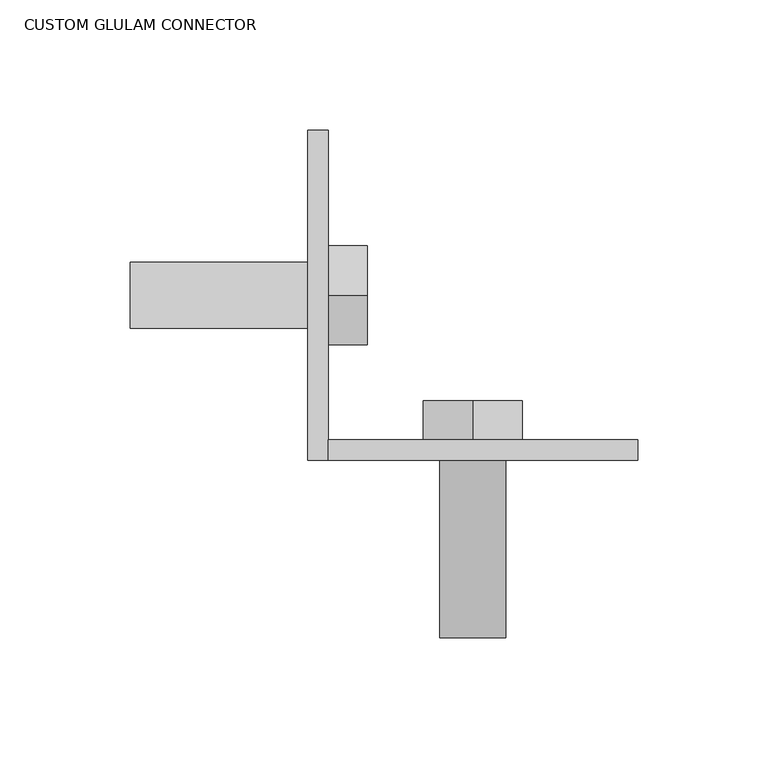
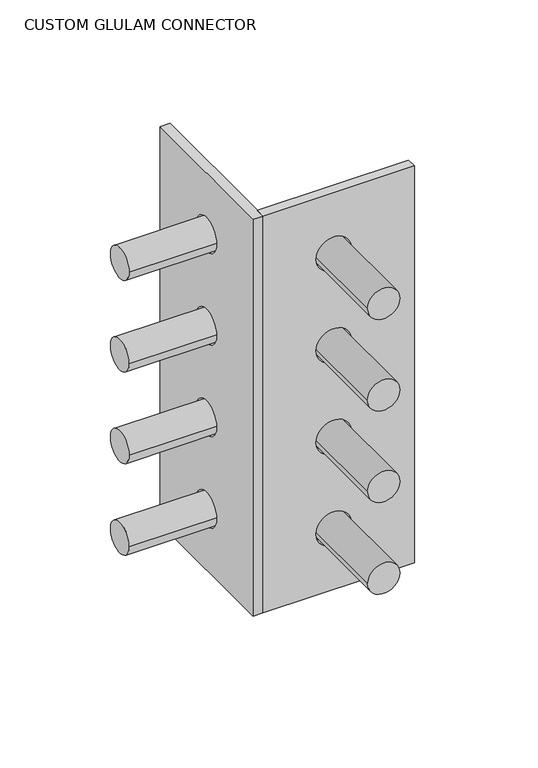
"""IFC4 building model written with IfcOpenShell, lengths in millimetres: fastener geometry, CUSTOM GLULAM CONNECTOR."""

from ifc_helpers import new_model, si_unit, point, frame, frame_2d, origin, place, context, project, spatial, polyline, circle_curve, trimmed, segment, composite_curve, outline, extrude, source, transform, mapped, element, save
from ifc_brep_helpers import plane_surface, revolved_surface, advanced_brep


def custom_glulam_connector_2ae8ac1e(model_context):
    return source(origin(), model_context, "Body", "SolidModel", [
        extrude(outline(polyline([(719.1375, 214.3125), (719.1375, 95.25), (388.9375, 95.25), (388.9375, 214.3125), (719.1375, 214.3125)]), holes=[composite_curve([segment(trimmed(circle_curve(frame_2d((592.1375, 150.8125)), 13.890625), [point((592.1375, 136.921875))], [point((592.1375, 164.703125))], True, "CARTESIAN"), True, "CONTINUOUS"), segment(trimmed(circle_curve(frame_2d((592.1375, 150.8125)), 13.890625), [point((592.1375, 164.703125))], [point((592.1375, 136.921875))], True, "CARTESIAN"), True, "CONTINUOUS")], self_intersect=False), composite_curve([segment(trimmed(circle_curve(frame_2d((668.3375, 150.8125)), 13.890625), [point((668.3375, 136.921875))], [point((668.3375, 164.703125))], True, "CARTESIAN"), True, "CONTINUOUS"), segment(trimmed(circle_curve(frame_2d((668.3375, 150.8125)), 13.890625), [point((668.3375, 164.703125))], [point((668.3375, 136.921875))], True, "CARTESIAN"), True, "CONTINUOUS")], self_intersect=False), composite_curve([segment(trimmed(circle_curve(frame_2d((515.9375, 150.8125)), 13.890625), [point((515.9375, 136.921875))], [point((515.9375, 164.703125))], True, "CARTESIAN"), True, "CONTINUOUS"), segment(trimmed(circle_curve(frame_2d((515.9375, 150.8125)), 13.890625), [point((515.9375, 164.703125))], [point((515.9375, 136.921875))], True, "CARTESIAN"), True, "CONTINUOUS")], self_intersect=False), composite_curve([segment(trimmed(circle_curve(frame_2d((439.7375, 150.8125)), 13.890625), [point((439.7375, 136.921875))], [point((439.7375, 164.703125))], True, "CARTESIAN"), True, "CONTINUOUS"), segment(trimmed(circle_curve(frame_2d((439.7375, 150.8125)), 13.890625), [point((439.7375, 164.703125))], [point((439.7375, 136.921875))], True, "CARTESIAN"), True, "CONTINUOUS")], self_intersect=False)]), frame((0.0, -63.5, 0.0), z_axis=(0.0, 1.0, 0.0), x_axis=(0.0, 0.0, 1.0)), (0.0, 0.0, 1.0), 7.9375),
        extrude(outline(polyline([(679.3360226, 131.7625), (657.3389774, 131.7625), (646.3404547, 150.8125), (657.3389774, 169.8625), (679.3360226, 169.8625), (690.3345453, 150.8125), (679.3360226, 131.7625)])), frame((0.0, -55.5625, 0.0), z_axis=(0.0, 1.0, 0.0), x_axis=(0.0, 0.0, 1.0)), (0.0, 0.0, 1.0), 14.9820312),
        extrude(outline(composite_curve([segment(trimmed(circle_curve(frame_2d((668.3375, 150.8125)), 12.7), [point((668.3375, 138.1125))], [point((668.3375, 163.5125))], False, "CARTESIAN"), True, "CONTINUOUS"), segment(trimmed(circle_curve(frame_2d((668.3375, 150.8125)), 12.7), [point((668.3375, 163.5125))], [point((668.3375, 138.1125))], False, "CARTESIAN"), True, "CONTINUOUS")], self_intersect=False)), frame((0.0, -131.7625, 0.0), z_axis=(0.0, 1.0, 0.0), x_axis=(0.0, 0.0, 1.0)), (0.0, 0.0, 1.0), 76.2),
        extrude(outline(polyline([(603.1360226, 131.7625), (581.1389774, 131.7625), (570.1404547, 150.8125), (581.1389774, 169.8625), (603.1360226, 169.8625), (614.1345453, 150.8125), (603.1360226, 131.7625)])), frame((0.0, -55.5625, 0.0), z_axis=(0.0, 1.0, 0.0), x_axis=(0.0, 0.0, 1.0)), (0.0, 0.0, 1.0), 14.9820312),
        extrude(outline(composite_curve([segment(trimmed(circle_curve(frame_2d((592.1375, 150.8125)), 12.7), [point((592.1375, 138.1125))], [point((592.1375, 163.5125))], False, "CARTESIAN"), True, "CONTINUOUS"), segment(trimmed(circle_curve(frame_2d((592.1375, 150.8125)), 12.7), [point((592.1375, 163.5125))], [point((592.1375, 138.1125))], False, "CARTESIAN"), True, "CONTINUOUS")], self_intersect=False)), frame((0.0, -131.7625, 0.0), z_axis=(0.0, 1.0, 0.0), x_axis=(0.0, 0.0, 1.0)), (0.0, 0.0, 1.0), 76.2),
        extrude(outline(polyline([(679.3360226, 131.7625), (657.3389774, 131.7625), (646.3404547, 150.8125), (657.3389774, 169.8625), (679.3360226, 169.8625), (690.3345453, 150.8125), (679.3360226, 131.7625)])), frame((0.0, -55.5625, 0.0), z_axis=(0.0, 1.0, 0.0), x_axis=(0.0, 0.0, 1.0)), (0.0, 0.0, 1.0), 14.9820312),
        extrude(outline(composite_curve([segment(trimmed(circle_curve(frame_2d((668.3375, 150.8125)), 12.7), [point((668.3375, 138.1125))], [point((668.3375, 163.5125))], False, "CARTESIAN"), True, "CONTINUOUS"), segment(trimmed(circle_curve(frame_2d((668.3375, 150.8125)), 12.7), [point((668.3375, 163.5125))], [point((668.3375, 138.1125))], False, "CARTESIAN"), True, "CONTINUOUS")], self_intersect=False)), frame((0.0, -131.7625, 0.0), z_axis=(0.0, 1.0, 0.0), x_axis=(0.0, 0.0, 1.0)), (0.0, 0.0, 1.0), 76.2),
        extrude(outline(polyline([(526.9360226, 131.7625), (504.9389774, 131.7625), (493.9404547, 150.8125), (504.9389774, 169.8625), (526.9360226, 169.8625), (537.9345453, 150.8125), (526.9360226, 131.7625)])), frame((0.0, -55.5625, 0.0), z_axis=(0.0, 1.0, 0.0), x_axis=(0.0, 0.0, 1.0)), (0.0, 0.0, 1.0), 14.9820312),
        extrude(outline(composite_curve([segment(trimmed(circle_curve(frame_2d((515.9375, 150.8125)), 12.7), [point((515.9375, 138.1125))], [point((515.9375, 163.5125))], False, "CARTESIAN"), True, "CONTINUOUS"), segment(trimmed(circle_curve(frame_2d((515.9375, 150.8125)), 12.7), [point((515.9375, 163.5125))], [point((515.9375, 138.1125))], False, "CARTESIAN"), True, "CONTINUOUS")], self_intersect=False)), frame((0.0, -131.7625, 0.0), z_axis=(0.0, 1.0, 0.0), x_axis=(0.0, 0.0, 1.0)), (0.0, 0.0, 1.0), 76.2),
        extrude(outline(polyline([(450.7360226, 131.7625), (428.7389774, 131.7625), (417.7404547, 150.8125), (428.7389774, 169.8625), (450.7360226, 169.8625), (461.7345453, 150.8125), (450.7360226, 131.7625)])), frame((0.0, -55.5625, 0.0), z_axis=(0.0, 1.0, 0.0), x_axis=(0.0, 0.0, 1.0)), (0.0, 0.0, 1.0), 14.9820312),
        extrude(outline(composite_curve([segment(trimmed(circle_curve(frame_2d((439.7375, 150.8125)), 12.7), [point((439.7375, 138.1125))], [point((439.7375, 163.5125))], False, "CARTESIAN"), True, "CONTINUOUS"), segment(trimmed(circle_curve(frame_2d((439.7375, 150.8125)), 12.7), [point((439.7375, 163.5125))], [point((439.7375, 138.1125))], False, "CARTESIAN"), True, "CONTINUOUS")], self_intersect=False)), frame((0.0, -131.7625, 0.0), z_axis=(0.0, 1.0, 0.0), x_axis=(0.0, 0.0, 1.0)), (0.0, 0.0, 1.0), 76.2),
        advanced_brep(
        [(95.25, -13.890625, 592.1375), (87.3125, -13.890625, 592.1375), (87.3125, 13.890625, 592.1375), (95.25, 13.890625, 592.1375), (95.25, -63.5, 719.1375), (95.25, -55.5625, 719.1375), (95.25, 63.5, 719.1375), (87.3125, 63.5, 719.1375), (87.3125, -63.5, 719.1375), (87.3125, 63.5, 388.9375), (87.3125, -63.5, 388.9375), (87.3125, -13.890625, 668.3375), (87.3125, 13.890625, 668.3375), (87.3125, -13.890625, 515.9375), (87.3125, 13.890625, 515.9375), (87.3125, -13.890625, 439.7375), (87.3125, 13.890625, 439.7375), (95.25, -63.5, 388.9375), (95.25, -55.5625, 388.9375), (95.25, 63.5, 388.9375), (95.25, 13.890625, 668.3375), (95.25, -13.890625, 668.3375), (95.25, 13.890625, 515.9375), (95.25, -13.890625, 515.9375), (95.25, 13.890625, 439.7375), (95.25, -13.890625, 439.7375)],
        [
            (0, 1),
            (1, 2, circle_curve(frame((87.3125, 0.0, 592.1375), z_axis=(-1.0, 0.0, 0.0), x_axis=(0.0, 1.0, 0.0)), 13.890625)),
            (2, 3),
            (3, 0, circle_curve(frame((95.25, 0.0, 592.1375), z_axis=(1.0, 0.0, 0.0), x_axis=(0.0, 1.0, 0.0)), 13.890625)),
            (4, 5),
            (5, 6),
            (6, 7),
            (7, 8),
            (8, 4),
            (7, 9),
            (9, 10),
            (10, 8),
            (11, 12, circle_curve(frame((87.3125, 0.0, 668.3375), z_axis=(1.0, 0.0, 0.0), x_axis=(0.0, 1.0, 0.0)), 13.890625)),
            (12, 11, circle_curve(frame((87.3125, 0.0, 668.3375), z_axis=(1.0, 0.0, 0.0), x_axis=(0.0, 1.0, 0.0)), 13.890625)),
            (1, 2, circle_curve(frame((87.3125, 0.0, 592.1375), z_axis=(1.0, 0.0, 0.0), x_axis=(0.0, 1.0, 0.0)), 13.890625)),
            (13, 14, circle_curve(frame((87.3125, 0.0, 515.9375), z_axis=(1.0, 0.0, 0.0), x_axis=(0.0, 1.0, 0.0)), 13.890625)),
            (14, 13, circle_curve(frame((87.3125, 0.0, 515.9375), z_axis=(1.0, 0.0, 0.0), x_axis=(0.0, 1.0, 0.0)), 13.890625)),
            (15, 16, circle_curve(frame((87.3125, 0.0, 439.7375), z_axis=(1.0, 0.0, 0.0), x_axis=(0.0, 1.0, 0.0)), 13.890625)),
            (16, 15, circle_curve(frame((87.3125, 0.0, 439.7375), z_axis=(1.0, 0.0, 0.0), x_axis=(0.0, 1.0, 0.0)), 13.890625)),
            (4, 17),
            (17, 18),
            (18, 19),
            (19, 6),
            (20, 21, circle_curve(frame((95.25, 0.0, 668.3375), z_axis=(-1.0, 0.0, 0.0), x_axis=(0.0, 1.0, 0.0)), 13.890625)),
            (21, 20, circle_curve(frame((95.25, 0.0, 668.3375), z_axis=(-1.0, 0.0, 0.0), x_axis=(0.0, 1.0, 0.0)), 13.890625)),
            (3, 0, circle_curve(frame((95.25, 0.0, 592.1375), z_axis=(-1.0, 0.0, 0.0), x_axis=(0.0, 1.0, 0.0)), 13.890625)),
            (22, 23, circle_curve(frame((95.25, 0.0, 515.9375), z_axis=(-1.0, 0.0, 0.0), x_axis=(0.0, 1.0, 0.0)), 13.890625)),
            (23, 22, circle_curve(frame((95.25, 0.0, 515.9375), z_axis=(-1.0, 0.0, 0.0), x_axis=(0.0, 1.0, 0.0)), 13.890625)),
            (24, 25, circle_curve(frame((95.25, 0.0, 439.7375), z_axis=(-1.0, 0.0, 0.0), x_axis=(0.0, 1.0, 0.0)), 13.890625)),
            (25, 24, circle_curve(frame((95.25, 0.0, 439.7375), z_axis=(-1.0, 0.0, 0.0), x_axis=(0.0, 1.0, 0.0)), 13.890625)),
            (10, 17),
            (19, 9),
            (11, 21),
            (20, 12),
            (23, 13),
            (14, 22),
            (25, 15),
            (16, 24),
        ],
        [
            revolved_surface(polyline([(95.25, 13.890625, 592.1375), (87.3125, 13.890625, 592.1375)]), (87.3125, 0.0, 592.1375), (1.0, 0.0, 0.0)),
            plane_surface(frame((95.25, 63.5, 719.1375), z_axis=(0.0, 0.0, 1.0), x_axis=(-1.0, 0.0, 0.0))),
            plane_surface(frame((87.3125, -63.5, 719.1375), z_axis=(-1.0, 0.0, 0.0), x_axis=(0.0, 1.0, 0.0))),
            plane_surface(frame((95.25, -63.5, 719.1375), z_axis=(1.0, 0.0, 0.0), x_axis=(0.0, -1.0, 0.0))),
            plane_surface(frame((95.25, -63.5, 719.1375), z_axis=(0.0, -1.0, 0.0), x_axis=(-1.0, 0.0, 0.0))),
            plane_surface(frame((95.25, 63.5, 388.9375), z_axis=(0.0, 1.0, 0.0), x_axis=(-1.0, 0.0, 0.0))),
            revolved_surface(polyline([(95.25, 13.890625, 668.3375), (87.3125, 13.890625, 668.3375)]), (87.3125, 0.0, 668.3375), (1.0, 0.0, 0.0)),
            plane_surface(frame((95.25, -63.5, 388.9375), z_axis=(0.0, 0.0, -1.0), x_axis=(-1.0, 0.0, 0.0))),
            revolved_surface(polyline([(95.25, 13.890625, 515.9375), (87.3125, 13.890625, 515.9375)]), (87.3125, 0.0, 515.9375), (1.0, 0.0, 0.0)),
            revolved_surface(polyline([(95.25, 13.890625, 439.7375), (87.3125, 13.890625, 439.7375)]), (87.3125, 0.0, 439.7375), (1.0, 0.0, 0.0)),
        ],
        [
            (0, [[1, 2, 3, 4]]),
            (1, [[5, 6, 7, 8, 9]]),
            (2, [[10, 11, 12, -8], [13, 14], [15, -2], [16, 17], [18, 19]]),
            (3, [[-6, -5, 20, 21, 22, 23], [24, 25], [26, -4], [27, 28], [29, 30]]),
            (4, [[-20, -9, -12, 31]]),
            (5, [[-23, 32, -10, -7]]),
            (6, [[33, -24, 34, -13]]),
            (6, [[-33, -14, -34, -25]]),
            (0, [[-1, -26, -3, -15]]),
            (7, [[-22, -21, -31, -11, -32]]),
            (8, [[35, -17, 36, -28]]),
            (9, [[37, -19, 38, -30]]),
            (9, [[-37, -29, -38, -18]]),
            (8, [[-35, -27, -36, -16]]),
        ],
    ),
        extrude(outline(polyline([(-19.05, 679.3360226), (0.0, 690.3345453), (19.05, 679.3360226), (19.05, 657.3389774), (0.0, 646.3404547), (-19.05, 657.3389774), (-19.05, 679.3360226)])), frame((95.25, 0.0, 0.0), z_axis=(1.0, 0.0, 0.0), x_axis=(0.0, 1.0, 0.0)), (0.0, 0.0, 1.0), 14.9820312),
        extrude(outline(composite_curve([segment(trimmed(circle_curve(frame_2d((0.0, 668.3375)), 12.7), [point((-12.7, 668.3375))], [point((12.7, 668.3375))], False, "CARTESIAN"), True, "CONTINUOUS"), segment(trimmed(circle_curve(frame_2d((0.0, 668.3375)), 12.7), [point((12.7, 668.3375))], [point((-12.7, 668.3375))], False, "CARTESIAN"), True, "CONTINUOUS")], self_intersect=False)), frame((19.05, 0.0, 0.0), z_axis=(1.0, 0.0, 0.0), x_axis=(0.0, 1.0, 0.0)), (0.0, 0.0, 1.0), 76.2),
        extrude(outline(polyline([(-19.05, 603.1360226), (0.0, 614.1345453), (19.05, 603.1360226), (19.05, 581.1389774), (0.0, 570.1404547), (-19.05, 581.1389774), (-19.05, 603.1360226)])), frame((95.25, 0.0, 0.0), z_axis=(1.0, 0.0, 0.0), x_axis=(0.0, 1.0, 0.0)), (0.0, 0.0, 1.0), 14.9820312),
        extrude(outline(composite_curve([segment(trimmed(circle_curve(frame_2d((0.0, 592.1375)), 12.7), [point((-12.7, 592.1375))], [point((12.7, 592.1375))], False, "CARTESIAN"), True, "CONTINUOUS"), segment(trimmed(circle_curve(frame_2d((0.0, 592.1375)), 12.7), [point((12.7, 592.1375))], [point((-12.7, 592.1375))], False, "CARTESIAN"), True, "CONTINUOUS")], self_intersect=False)), frame((19.05, 0.0, 0.0), z_axis=(1.0, 0.0, 0.0), x_axis=(0.0, 1.0, 0.0)), (0.0, 0.0, 1.0), 76.2),
        extrude(outline(polyline([(-19.05, 679.3360226), (0.0, 690.3345453), (19.05, 679.3360226), (19.05, 657.3389774), (0.0, 646.3404547), (-19.05, 657.3389774), (-19.05, 679.3360226)])), frame((95.25, 0.0, 0.0), z_axis=(1.0, 0.0, 0.0), x_axis=(0.0, 1.0, 0.0)), (0.0, 0.0, 1.0), 14.9820312),
        extrude(outline(composite_curve([segment(trimmed(circle_curve(frame_2d((0.0, 668.3375)), 12.7), [point((-12.7, 668.3375))], [point((12.7, 668.3375))], False, "CARTESIAN"), True, "CONTINUOUS"), segment(trimmed(circle_curve(frame_2d((0.0, 668.3375)), 12.7), [point((12.7, 668.3375))], [point((-12.7, 668.3375))], False, "CARTESIAN"), True, "CONTINUOUS")], self_intersect=False)), frame((19.05, 0.0, 0.0), z_axis=(1.0, 0.0, 0.0), x_axis=(0.0, 1.0, 0.0)), (0.0, 0.0, 1.0), 76.2),
        extrude(outline(polyline([(-19.05, 526.9360226), (0.0, 537.9345453), (19.05, 526.9360226), (19.05, 504.9389774), (0.0, 493.9404547), (-19.05, 504.9389774), (-19.05, 526.9360226)])), frame((95.25, 0.0, 0.0), z_axis=(1.0, 0.0, 0.0), x_axis=(0.0, 1.0, 0.0)), (0.0, 0.0, 1.0), 14.9820312),
        extrude(outline(composite_curve([segment(trimmed(circle_curve(frame_2d((0.0, 515.9375)), 12.7), [point((-12.7, 515.9375))], [point((12.7, 515.9375))], False, "CARTESIAN"), True, "CONTINUOUS"), segment(trimmed(circle_curve(frame_2d((0.0, 515.9375)), 12.7), [point((12.7, 515.9375))], [point((-12.7, 515.9375))], False, "CARTESIAN"), True, "CONTINUOUS")], self_intersect=False)), frame((19.05, 0.0, 0.0), z_axis=(1.0, 0.0, 0.0), x_axis=(0.0, 1.0, 0.0)), (0.0, 0.0, 1.0), 76.2),
        extrude(outline(polyline([(-19.05, 450.7360226), (0.0, 461.7345453), (19.05, 450.7360226), (19.05, 428.7389774), (0.0, 417.7404547), (-19.05, 428.7389774), (-19.05, 450.7360226)])), frame((95.25, 0.0, 0.0), z_axis=(1.0, 0.0, 0.0), x_axis=(0.0, 1.0, 0.0)), (0.0, 0.0, 1.0), 14.9820312),
        extrude(outline(composite_curve([segment(trimmed(circle_curve(frame_2d((0.0, 439.7375)), 12.7), [point((-12.7, 439.7375))], [point((12.7, 439.7375))], False, "CARTESIAN"), True, "CONTINUOUS"), segment(trimmed(circle_curve(frame_2d((0.0, 439.7375)), 12.7), [point((12.7, 439.7375))], [point((-12.7, 439.7375))], False, "CARTESIAN"), True, "CONTINUOUS")], self_intersect=False)), frame((19.05, 0.0, 0.0), z_axis=(1.0, 0.0, 0.0), x_axis=(0.0, 1.0, 0.0)), (0.0, 0.0, 1.0), 76.2),
    ])


if __name__ == "__main__":
    model = new_model("IFC4")
    model_context = context("Model", 3, world=origin())
    ifc_project = project(units=[si_unit("LENGTHUNIT", "METRE", prefix="MILLI")], contexts=[model_context])
    site = spatial("IfcSite", under=ifc_project)
    building = spatial("IfcBuilding", under=site)
    placement = place(None, origin())
    custom_glulam_connector_shape = custom_glulam_connector_2ae8ac1e(model_context)
    element("IfcFastener", 1, ObjectType="CUSTOM GLULAM CONNECTOR : CUSTOM - L5\"x5\"x5/16\"x13\" - HDG", at=placement, inside=building, context=model_context, shape_type="MappedRepresentation", body=[
        mapped(custom_glulam_connector_shape, transform((0.0, 0.0, 0.0), x_axis=(1.0, 0.0, 0.0), y_axis=(0.0, 1.0, 0.0), z_axis=(0.0, 0.0, 1.0))),
    ])
    save(model, "model.ifc")

# Revit data of these elements
# Type "CUSTOM GLULAM CONNECTOR : CUSTOM - L5\"x5\"x5/16\"x13\" - HDG"
#   Width - Top = 0' - 6 7/8"
#   Top/Bottom Plate Thickness = 0' - 0 5/16"
#   Top/Bottom Plate - Width = 0' - 7 1/2"
#   Rod Radius = 0' - 0 1/2"
#   Rod Length [instance default] = 1' - 0"
#   Plate Thickness = 0' - 0 5/16"
#   Offset - Upper Plate 2 = 0' - 0"
#   Height of Plate = 1' - 3"
#   Width - Bottom = 0' - 6 7/8"
#   Plate Width = 0' - 5"
#   Bracket Width = 0' - 5 1/4"
#   Bracket Thickness = 0' - 0 5/8"
#   Bracket Offset in X = 0' - 3 3/4"
#   Bracket Offset in Y = 0' - 0 3/4"
#   Bracket Offset = 0' - 1 1/2"
#   Bracket Leg = 0' - 8"
#   Bracket Hole Radius - Up = 0' - 0 1/2"
#   Bracket Hole Radius - Down = 0' - 0 1/2"
#   Bracket Hole Offset = 0' - 2"
#   Beam Width = 0' - 7 3/8"
#   Angle 2 = 61.00°
#   Angle 1 = 151.00°
#   Top Plate Visible = no
#   Rod Visibility = no
#   Plate Visibility - Upper Right 2 = yes
#   Plate Visibility - Upper Right 1 = yes
#   Plate Visibility - Upper Left 2 = no
#   Plate Visibility - Upper Left 1 = no
#   Plate Visibility - Lower Right 2 = no
#   Plate Visibility - Lower Right 1 = no
#   Plate Visibility - Lower Left 2 = no
#   Plate Visibility - Lower Left 1 = no
#   Bracket Visibility = no
#   Bottom Plate Visible = no
#   Upper Plates - 2 = element 1868899
#   Upper Plates - 1 = element 1868901
#   Lower Plates = element 1746392
#   Bracket Material = L5"x5"x5/16" STEEL ANGLE (HDG AFTER FABRICATION)
#   URL = ""
# Element 1 (IfcFastener, "CUSTOM GLULAM CONNECTOR : CUSTOM - L5\"x5\"x5/16\"x13\" - HDG")
#   Materials on its faces: "1\" GALV. LAG BOLT (LENGTH = 1/2\" SHY OF GLULAM DEPTH) -  (GALV. THRU BOLT IF PLATE ON OPP. SIDE OF STRUCT MEMBER)", "L5\"x5\"x5/16\" STEEL ANGLE (HDG AFTER FABRICATION)"
# Materials
#   "L5\"x5\"x5/16\" STEEL ANGLE (HDG AFTER FABRICATION)": class "Generic", colour RGB 232 232 232, transparency 0, Cost = 0
#   "1\" GALV. LAG BOLT (LENGTH = 1/2\" SHY OF GLULAM DEPTH) -  (GALV. THRU BOLT IF PLATE ON OPP. SIDE OF STRUCT MEMBER)": class "Generic", colour RGB 120 120 120, transparency 0, Cost = 0
